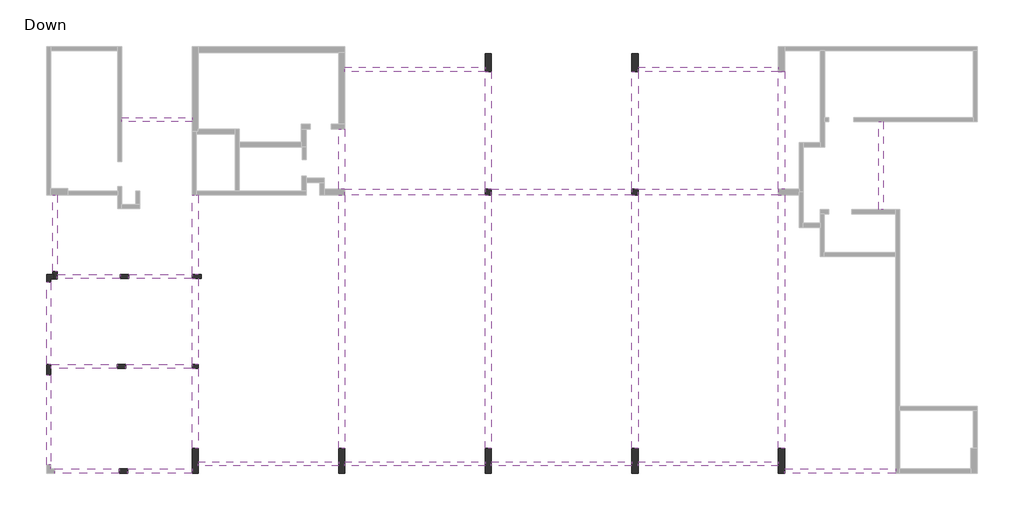
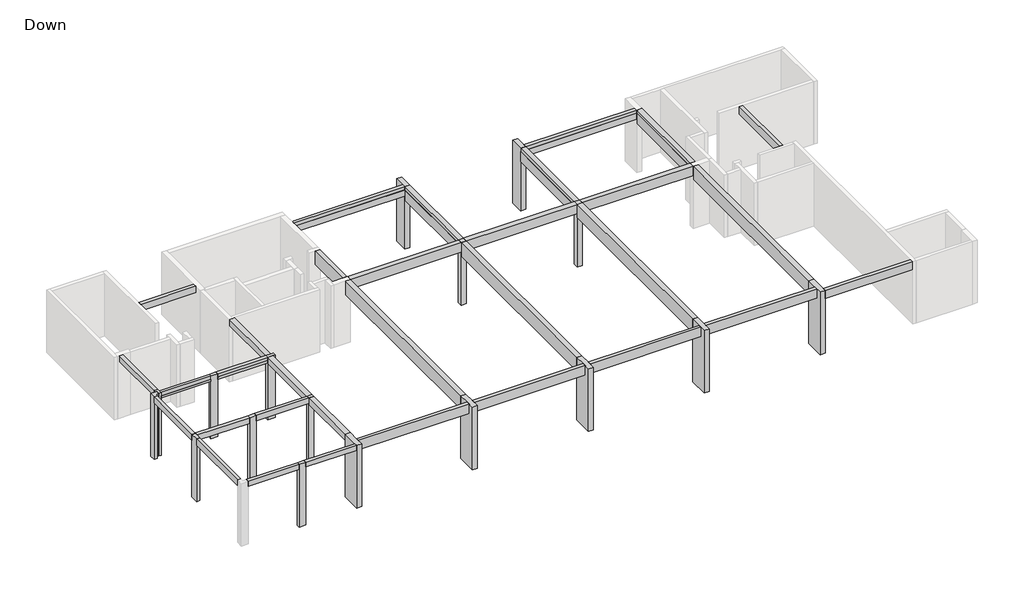
# One storey, part 2 of 2: 32 beams, 17 columns.
"""IFC4 building model written with IfcOpenShell, lengths in millimetres."""

from ifc_helpers import new_model, si_unit, frame, origin, origin_with_axes, place, context, project, spatial, polyline, outline, extrude, faceted_brep, element, save

model = new_model("IFC4")

# Units and contexts
model_context = context("Model", 3, world=origin())
ifc_project = project(units=[si_unit("LENGTHUNIT", "METRE", prefix="MILLI")], contexts=[model_context])

# Site, building, storey
site = spatial("IfcSite", under=ifc_project)
building = spatial("IfcBuilding", under=site)
storey = spatial("IfcBuildingStorey", under=building, Name="Down", Elevation=0.0)

# Beams
placement = place(None, origin())
element("IfcBeam", 1, ObjectType="Concrete Rectengular Beam : 20/30", at=placement, inside=storey, context=model_context, shape_type="Brep", body=[
    faceted_brep([(-13943.2656756, 4006.6682295, 4000.0), (-13943.2656756, 4206.6682295, 4000.0), (-17016.9438365, 4206.6682295, 4000.0), (-17016.9438365, 4006.6682295, 4000.0), (-13943.2656756, 4006.6682295, 3700.0), (-17016.9438365, 4006.6682295, 3700.0), (-13943.2656756, 4206.6682295, 3700.0), (-17016.9438365, 4206.6682295, 3700.0), (-13943.2656756, 4206.6682295, 3790.0)], [[[0, 1, 2, 3]], [[4, 0, 3, 5]], [[6, 4, 5, 7]], [[1, 8, 6, 7, 2]], [[1, 0, 4, 6, 8]], [[3, 2, 7, 5]]]),
])
element("IfcBeam", 2, ObjectType="Concrete Rectengular Beam : 20/30", at=placement, inside=storey, context=model_context, shape_type="SweptSolid", body=[
    extrude(outline(polyline([(-17416.9438365, 4206.6682295), (-17416.9438365, 4006.6682295), (-20492.8250626, 4006.6682295), (-20492.8250626, 4206.6682295), (-17416.9438365, 4206.6682295)])), frame((0.0, 0.0, 3700.0), z_axis=(0.0, 0.0, 1.0), x_axis=(1.0, 0.0, 0.0)), (0.0, 0.0, 1.0), 300.0),
])
element("IfcBeam", 3, ObjectType="Concrete Rectengular Beam : 20/35", at=placement, inside=storey, context=model_context, shape_type="Brep", body=[
    faceted_brep([(-17368.3423039, 13503.9096088, 4000.0), (-20386.1465057, 13503.9096088, 4000.0), (-20386.1465057, 13308.9096088, 4000.0), (-17368.3423039, 13308.9096088, 4000.0), (-20386.1465057, 13303.9096088, 3650.0), (-17368.3423039, 13303.9096088, 3650.0), (-17368.3423039, 13303.9096088, 3790.0), (-20386.1465057, 13303.9096088, 3790.0), (-17368.3423039, 13503.9096088, 3650.0), (-20386.1465057, 13503.9096088, 3650.0), (-20386.1465057, 13503.9096088, 3790.0), (-17368.3423039, 13308.9096088, 3790.0), (-20386.1465057, 13308.9096088, 3790.0)], [[[0, 1, 2, 3]], [[4, 5, 6, 7]], [[8, 5, 4, 9]], [[0, 8, 9, 10, 1]], [[5, 8, 0, 3, 11, 6]], [[9, 4, 7, 12, 2, 1, 10]], [[11, 12, 7, 6]], [[12, 11, 3, 2]]]),
])
element("IfcBeam", 4, ObjectType="Concrete Rectengular Beam : 20/35", at=placement, inside=storey, context=model_context, shape_type="SweptSolid", body=[
    extrude(outline(polyline([(13503.9096088, 3650.0), (13303.9096088, 3650.0), (13303.9096088, 3790.0), (13308.9096088, 3790.0), (13308.9096088, 4000.0), (13503.9096088, 4000.0), (13503.9096088, 3650.0)])), frame((-16968.3423039, 0.0, 0.0), z_axis=(1.0, 0.0, 0.0), x_axis=(0.0, 1.0, 0.0)), (0.0, 0.0, 1.0), 3023.8505747),
])
element("IfcBeam", 5, ObjectType="Concrete Rectengular Beam : 20/35", at=placement, inside=storey, context=model_context, shape_type="Brep", body=[
    faceted_brep([(-20586.1465057, 13648.5145478, 4000.0), (-20386.1465057, 13648.5145478, 4000.0), (-20386.1465057, 17305.3655475, 4000.0), (-20586.1465057, 17305.3655475, 4000.0), (-20386.1465057, 13648.5145478, 3650.0), (-20386.1465057, 17305.3655475, 3650.0), (-20386.1465057, 17305.3655475, 3790.0), (-20586.1465057, 13648.5145478, 3650.0), (-20586.1465057, 17305.3655475, 3650.0)], [[[0, 1, 2, 3]], [[1, 4, 5, 6, 2]], [[4, 7, 8, 5]], [[7, 0, 3, 8]], [[1, 0, 7, 4]], [[3, 2, 6, 5, 8]]]),
])
element("IfcBeam", 6, ObjectType="Concrete Rectengular Beam : 20/35", at=placement, inside=storey, context=model_context, shape_type="SweptSolid", body=[
    extrude(outline(polyline([(-20678.0944112, 9006.6873866), (-20678.0944112, 9206.6873866), (-17516.5223806, 9206.6873866), (-17516.5223806, 9006.6873866), (-20678.0944112, 9006.6873866)])), frame((0.0, 0.0, 3650.0), z_axis=(0.0, 0.0, 1.0), x_axis=(1.0, 0.0, 0.0)), (0.0, 0.0, 1.0), 350.0),
])
element("IfcBeam", 7, ObjectType="Concrete Rectengular Beam : 20/35", at=placement, inside=storey, context=model_context, shape_type="Brep", body=[
    faceted_brep([(-17116.5223806, 9206.6873866, 4000.0), (-17116.5223806, 9006.6873866, 4000.0), (-13943.2656756, 9006.6873866, 4000.0), (-13943.2656756, 9206.6873866, 4000.0), (-17116.5223806, 9006.6873866, 3650.0), (-13943.2656756, 9006.6873866, 3650.0), (-13943.2656756, 9006.6873866, 3790.0), (-17116.5223806, 9206.6873866, 3650.0), (-13943.2656756, 9206.6873866, 3650.0), (-13943.2656756, 9206.6873866, 3790.0)], [[[0, 1, 2, 3]], [[1, 4, 5, 6, 2]], [[4, 7, 8, 5]], [[7, 0, 3, 9, 8]], [[1, 0, 7, 4]], [[2, 6, 5, 8, 9, 3]]]),
])
element("IfcBeam", 8, ObjectType="Concrete Rectengular Beam : 20/40", at=placement, inside=storey, context=model_context, shape_type="Brep", body=[
    faceted_brep([(-20690.7944112, 9206.6873866, 4000.0), (-20890.7944112, 9206.6873866, 4000.0), (-20890.7944112, 9205.6720609, 4000.0), (-20690.7944112, 9205.6720609, 4000.0), (-20690.7944112, 9206.6873866, 3600.0), (-20690.7944112, 9205.6720609, 3600.0), (-20890.7944112, 9206.6873866, 3600.0), (-20890.7944112, 9205.6720609, 3600.0)], [[[0, 1, 2, 3]], [[4, 0, 3, 5]], [[6, 4, 5, 7]], [[1, 6, 7, 2]], [[1, 0, 4, 6]], [[3, 2, 7, 5]]]),
    faceted_brep([(-20890.7944112, 8705.6720609, 4000.0), (-20690.7944112, 8705.6720609, 4000.0), (-20690.7944112, 8705.6720609, 3600.0), (-20890.7944112, 8705.6720609, 3600.0), (-20692.8250626, 4406.6682295, 3600.0), (-20692.8250626, 4406.6682295, 4000.0), (-20890.7944112, 4406.6682295, 4000.0), (-20890.7944112, 4406.6682295, 3600.0), (-20692.8250626, 4206.6682295, 3600.0), (-20692.8250626, 4206.6682295, 4000.0), (-20690.7944112, 4206.6682295, 3600.0), (-20690.7944112, 4206.6682295, 3790.0), (-20690.7944112, 4206.6682295, 4000.0)], [[[0, 1, 2, 3]], [[4, 5, 6, 7]], [[5, 4, 8, 9]], [[9, 8, 10, 11, 12]], [[1, 0, 6, 5, 9, 12]], [[2, 1, 12, 11, 10]], [[3, 2, 10, 8, 4, 7]], [[0, 3, 7, 6]]]),
])
element("IfcBeam", 9, ObjectType="Concrete Rectengular Beam : 20/40", at=placement, inside=storey, context=model_context, shape_type="Brep", body=[
    faceted_brep([(-20890.7944112, 9206.6873866, 4000.0), (-20690.7944112, 9206.6873866, 4000.0), (-20690.7944112, 13148.3800933, 4000.0), (-20890.7944112, 13148.3800933, 4000.0), (-20690.7944112, 9206.6873866, 3790.0), (-20690.7944112, 9206.6873866, 3600.0), (-20690.7944112, 13148.3800933, 3600.0), (-20890.7944112, 9206.6873866, 3600.0), (-20890.7944112, 13148.3800933, 3600.0)], [[[0, 1, 2, 3]], [[1, 4, 5, 6, 2]], [[5, 7, 8, 6]], [[7, 0, 3, 8]], [[3, 2, 6, 8]], [[1, 0, 7, 5, 4]]]),
])
element("IfcBeam", 10, ObjectType="Concrete Rectengular Beam : 20/40", at=placement, inside=storey, context=model_context, shape_type="Brep", body=[
    faceted_brep([(-17292.1354074, 21006.0552027, 4000.0), (-17292.1354074, 20806.0552027, 4000.0), (-13943.2656756, 20806.0552027, 4000.0), (-13943.2656756, 21006.0552027, 4000.0), (-17292.1354074, 20806.0552027, 3790.0), (-17292.1354074, 20806.0552027, 3600.0), (-13943.2656756, 20806.0552027, 3600.0), (-13943.2656756, 20806.0552027, 3790.0), (-17292.1354074, 21006.0552027, 3600.0), (-13943.2656756, 21006.0552027, 3600.0)], [[[0, 1, 2, 3]], [[1, 4, 5, 6, 7, 2]], [[5, 8, 9, 6]], [[8, 0, 3, 9]], [[1, 0, 8, 5, 4]], [[3, 2, 7, 6, 9]]]),
])
element("IfcBeam", 11, ObjectType="Concrete Rectengular Beam : 20/50", at=placement, inside=storey, context=model_context, shape_type="Brep", body=[
    faceted_brep([(14358.5350907, 4204.8099919, 4000.0), (14358.5350907, 4004.8099919, 4000.0), (19658.7266616, 4004.8099919, 4000.0), (19658.7266616, 4204.8099919, 4000.0), (14358.5350907, 4004.8099919, 3500.0), (19658.7266616, 4004.8099919, 3500.0), (14358.5350907, 4204.8099919, 3500.0), (19658.7266616, 4204.8099919, 3500.0), (14358.5350907, 4204.8099919, 3790.0), (19658.7266616, 4204.8099919, 3790.0)], [[[0, 1, 2, 3]], [[1, 4, 5, 2]], [[4, 6, 7, 5]], [[6, 8, 0, 3, 9, 7]], [[1, 0, 8, 6, 4]], [[3, 2, 5, 7, 9]]]),
])
element("IfcBeam", 12, ObjectType="Concrete Rectengular Beam : 20/50", at=placement, inside=storey, context=model_context, shape_type="SweptSolid", body=[
    extrude(outline(polyline([(18864.3013742, 20804.7142065), (19064.3013742, 20804.7142065), (19064.3013742, 16606.2084594), (18864.3013742, 16606.2084594), (18864.3013742, 20804.7142065)])), frame((0.0, 0.0, 3500.0), z_axis=(0.0, 0.0, 1.0), x_axis=(1.0, 0.0, 0.0)), (0.0, 0.0, 1.0), 500.0),
])
element("IfcBeam", 13, ObjectType="Concrete Rectengular Beam : 20/60", at=placement, inside=storey, context=model_context, shape_type="Brep", body=[
    faceted_brep([(58.2285773, 23405.5571184, 4000.0), (-6644.3384725, 23405.5571184, 4000.0), (-6644.3384725, 23225.5571184, 4000.0), (58.2285773, 23225.5571184, 4000.0), (58.2285773, 23405.5571184, 3400.0), (-6644.3384725, 23405.5571184, 3400.0), (58.2285773, 23205.5571184, 3400.0), (-6644.3384725, 23205.5571184, 3400.0), (58.2285773, 23205.5571184, 3790.0), (-6644.3384725, 23205.5571184, 3790.0), (58.2285773, 23225.5571184, 3790.0), (58.2285773, 23206.5724441, 3790.0), (-6644.3384725, 23225.5571184, 3790.0)], [[[0, 1, 2, 3]], [[0, 4, 5, 1]], [[4, 6, 7, 5]], [[7, 6, 8, 9]], [[4, 0, 3, 10, 11, 8, 6]], [[1, 5, 7, 9, 12, 2]], [[10, 12, 9, 8, 11]], [[12, 10, 3, 2]]]),
])
element("IfcBeam", 14, ObjectType="Concrete Rectengular Beam : 20/60", at=placement, inside=storey, context=model_context, shape_type="Brep", body=[
    faceted_brep([(14058.5350907, 23405.5571184, 4000.0), (7356.7343244, 23405.5571184, 4000.0), (7356.7343244, 23210.5571184, 4000.0), (14058.5350907, 23210.5571184, 4000.0), (14358.5350907, 23205.5571184, 3400.0), (14358.5350907, 23205.5571184, 4000.0), (14063.5350907, 23205.5571184, 4000.0), (14063.5350907, 23205.5571184, 3790.0), (14058.5350907, 23205.5571184, 3790.0), (7356.7343244, 23205.5571184, 3790.0), (7356.7343244, 23205.5571184, 3400.0), (14058.5350907, 23205.5571184, 3400.0), (7356.7343244, 23405.5571184, 3400.0), (14058.5350907, 23405.5571184, 3400.0), (14058.5350907, 23206.5724441, 3400.0), (14358.5350907, 23206.5724441, 3400.0), (14358.5350907, 23206.5724441, 4000.0), (7356.7343244, 23206.5724441, 3790.0), (7356.7343244, 23210.5571184, 3790.0), (14058.5350907, 23210.5571184, 3790.0), (14058.5350907, 23206.5724441, 3790.0), (14063.5350907, 23206.5724441, 3790.0), (14063.5350907, 23206.5724441, 4000.0)], [[[0, 1, 2, 3]], [[4, 5, 6, 7, 8, 9, 10, 11]], [[4, 11, 10, 12, 13, 14, 15]], [[12, 1, 0, 13]], [[5, 4, 15, 16]], [[12, 10, 9, 17, 18, 2, 1]], [[14, 13, 0, 3, 19, 20]], [[15, 14, 20, 21, 22, 16]], [[19, 18, 17, 9, 8, 7, 21, 20]], [[21, 7, 6, 22]], [[18, 19, 3, 2]], [[5, 16, 22, 6]]]),
])
element("IfcBeam", 15, ObjectType="Concrete Rectengular Beam : 20/60", at=placement, inside=storey, context=model_context, shape_type="Brep", body=[
    faceted_brep([(7356.7343244, 4552.8176548, 4000.0), (7356.7343244, 4352.8176548, 4000.0), (14058.5350907, 4352.8176548, 4000.0), (14058.5350907, 4552.8176548, 4000.0), (7356.7343244, 4352.8176548, 3400.0), (14058.5350907, 4352.8176548, 3400.0), (7356.7343244, 4552.8176548, 3400.0), (14058.5350907, 4552.8176548, 3400.0), (7356.7343244, 4552.8176548, 3790.0), (14058.5350907, 4552.8176548, 3790.0)], [[[0, 1, 2, 3]], [[1, 4, 5, 2]], [[4, 6, 7, 5]], [[6, 8, 0, 3, 9, 7]], [[1, 0, 8, 6, 4]], [[3, 2, 5, 7, 9]]]),
])
element("IfcBeam", 16, ObjectType="Concrete Rectengular Beam : 20/60", at=placement, inside=storey, context=model_context, shape_type="Brep", body=[
    faceted_brep([(358.2285773, 4552.8176548, 4000.0), (358.2285773, 4352.8176548, 4000.0), (7056.7343244, 4352.8176548, 4000.0), (7056.7343244, 4552.8176548, 4000.0), (358.2285773, 4552.8176548, 3400.0), (358.2285773, 4552.8176548, 3790.0), (7056.7343244, 4552.8176548, 3790.0), (7056.7343244, 4552.8176548, 3400.0), (358.2285773, 4352.8176548, 3400.0), (7056.7343244, 4352.8176548, 3400.0)], [[[0, 1, 2, 3]], [[4, 5, 0, 3, 6, 7]], [[8, 4, 7, 9]], [[1, 8, 9, 2]], [[1, 0, 5, 4, 8]], [[3, 2, 9, 7, 6]]]),
])
element("IfcBeam", 17, ObjectType="Concrete Rectengular Beam : 20/60", at=placement, inside=storey, context=model_context, shape_type="Brep", body=[
    faceted_brep([(-6644.3384725, 4552.8176548, 4000.0), (-6644.3384725, 4352.8176548, 4000.0), (58.2285773, 4352.8176548, 4000.0), (58.2285773, 4552.8176548, 4000.0), (-6644.3384725, 4552.8176548, 3400.0), (-6644.3384725, 4552.8176548, 3790.0), (58.2285773, 4552.8176548, 3790.0), (58.2285773, 4552.8176548, 3400.0), (-6644.3384725, 4352.8176548, 3400.0), (58.2285773, 4352.8176548, 3400.0)], [[[0, 1, 2, 3]], [[4, 5, 0, 3, 6, 7]], [[8, 4, 7, 9]], [[1, 8, 9, 2]], [[1, 0, 5, 4, 8]], [[3, 2, 9, 7, 6]]]),
])
element("IfcBeam", 18, ObjectType="Concrete Rectengular Beam : 20/60", at=placement, inside=storey, context=model_context, shape_type="Brep", body=[
    faceted_brep([(-13643.2656756, 4552.8176548, 4000.0), (-13643.2656756, 4352.8176548, 4000.0), (-6944.3384725, 4352.8176548, 4000.0), (-6944.3384725, 4552.8176548, 4000.0), (-13643.2656756, 4552.8176548, 3400.0), (-13643.2656756, 4552.8176548, 3790.0), (-6944.3384725, 4552.8176548, 3790.0), (-6944.3384725, 4552.8176548, 3400.0), (-13643.2656756, 4352.8176548, 3400.0), (-6944.3384725, 4352.8176548, 3400.0)], [[[0, 1, 2, 3]], [[4, 5, 0, 3, 6, 7]], [[8, 4, 7, 9]], [[1, 8, 9, 2]], [[1, 0, 5, 4, 8]], [[3, 2, 9, 7, 6]]]),
])
element("IfcBeam", 19, ObjectType="Concrete Rectengular Beam : 30/40", at=placement, inside=storey, context=model_context, shape_type="Brep", body=[
    faceted_brep([(-13943.2656756, 13503.9096088, 4000.0), (-13643.2656756, 13503.9096088, 4000.0), (-13643.2656756, 17304.7716778, 4000.0), (-13743.2656756, 17304.7716778, 4000.0), (-13943.2656756, 17304.7716778, 4000.0), (-13643.2656756, 13503.9096088, 3790.0), (-13643.2656756, 13503.9096088, 3600.0), (-13643.2656756, 17304.7716778, 3600.0), (-13643.2656756, 17304.7716778, 3790.0), (-13943.2656756, 13503.9096088, 3600.0), (-13943.2656756, 17304.7716778, 3600.0), (-13943.2656756, 13503.9096088, 3790.0)], [[[0, 1, 2, 3, 4]], [[1, 5, 6, 7, 8, 2]], [[6, 9, 10, 7]], [[9, 11, 0, 4, 10]], [[1, 0, 11, 9, 6, 5]], [[2, 8, 7, 10, 4, 3]]]),
])
element("IfcBeam", 20, ObjectType="Concrete Rectengular Beam : 30/40", at=placement, inside=storey, context=model_context, shape_type="Brep", body=[
    faceted_brep([(-13643.2656756, 13303.9096088, 4000.0), (-13943.2656756, 13303.9096088, 4000.0), (-13943.2656756, 9206.6873866, 4000.0), (-13643.2656756, 9206.6873866, 4000.0), (-13943.2656756, 13303.9096088, 3790.0), (-13943.2656756, 13303.9096088, 3600.0), (-13943.2656756, 9206.6873866, 3600.0), (-13943.2656756, 9206.6873866, 3790.0), (-13643.2656756, 13303.9096088, 3600.0), (-13643.2656756, 9206.6873866, 3600.0), (-13643.2656756, 13303.9096088, 3790.0)], [[[0, 1, 2, 3]], [[1, 4, 5, 6, 7, 2]], [[5, 8, 9, 6]], [[8, 10, 0, 3, 9]], [[8, 5, 4, 1, 0, 10]], [[3, 2, 7, 6, 9]]]),
])
element("IfcBeam", 21, ObjectType="Concrete Rectengular Beam : 30/40", at=placement, inside=storey, context=model_context, shape_type="Brep", body=[
    faceted_brep([(-13943.2656756, 5204.8099919, 4000.0), (-13643.2656756, 5204.8099919, 4000.0), (-13643.2656756, 9006.6873866, 4000.0), (-13943.2656756, 9006.6873866, 4000.0), (-13943.2656756, 5204.8099919, 3600.0), (-13943.2656756, 9006.6873866, 3790.0), (-13943.2656756, 9006.6873866, 3600.0), (-13643.2656756, 5204.8099919, 3600.0), (-13643.2656756, 9006.6873866, 3600.0)], [[[0, 1, 2, 3]], [[4, 0, 3, 5, 6]], [[7, 4, 6, 8]], [[1, 7, 8, 2]], [[1, 0, 4, 7]], [[3, 2, 8, 6, 5]]]),
])
element("IfcBeam", 22, ObjectType="Concrete Rectengular Beam : 30/60", at=placement, inside=storey, context=model_context, shape_type="Brep", body=[
    faceted_brep([(-6644.3384725, 17297.4228975, 4000.0), (58.2285773, 17297.4228975, 4000.0), (58.2285773, 17587.4228975, 4000.0), (-6644.3384725, 17587.4228975, 4000.0), (58.2285773, 17297.4228975, 3400.0), (58.2285773, 17297.4228975, 3790.0), (-6644.3384725, 17297.4228975, 3790.0), (-6644.3384725, 17297.4228975, 3400.0), (58.2285773, 17597.4228975, 3400.0), (-6644.3384725, 17597.4228975, 3400.0), (-6644.3384725, 17597.4228975, 3790.0), (58.2285773, 17597.4228975, 3790.0), (58.2285773, 17587.4228975, 3790.0), (-6644.3384725, 17587.4228975, 3790.0)], [[[0, 1, 2, 3]], [[4, 5, 1, 0, 6, 7]], [[8, 4, 7, 9]], [[8, 9, 10, 11]], [[1, 5, 4, 8, 11, 12, 2]], [[7, 6, 0, 3, 13, 10, 9]], [[13, 12, 11, 10]], [[12, 13, 3, 2]]]),
])
element("IfcBeam", 23, ObjectType="Concrete Rectengular Beam : 30/60", at=placement, inside=storey, context=model_context, shape_type="Brep", body=[
    faceted_brep([(358.2285773, 17597.4228975, 4000.0), (358.2285773, 17297.4228975, 4000.0), (7056.7343244, 17297.4228975, 4000.0), (7056.7343244, 17597.4228975, 4000.0), (358.2285773, 17297.4228975, 3790.0), (358.2285773, 17297.4228975, 3400.0), (7056.7343244, 17297.4228975, 3400.0), (7056.7343244, 17297.4228975, 3790.0), (358.2285773, 17597.4228975, 3400.0), (7056.7343244, 17597.4228975, 3400.0)], [[[0, 1, 2, 3]], [[1, 4, 5, 6, 7, 2]], [[5, 8, 9, 6]], [[8, 0, 3, 9]], [[5, 4, 1, 0, 8]], [[2, 7, 6, 9, 3]]]),
])
element("IfcBeam", 24, ObjectType="Concrete Rectengular Beam : 30/60", at=placement, inside=storey, context=model_context, shape_type="Brep", body=[
    faceted_brep([(7356.7343244, 17297.4228975, 4000.0), (14058.5350907, 17297.4228975, 4000.0), (14058.5350907, 17587.4228975, 4000.0), (7356.7343244, 17587.4228975, 4000.0), (7356.7343244, 17297.4228975, 3790.0), (7356.7343244, 17297.4228975, 3400.0), (14058.5350907, 17297.4228975, 3400.0), (14058.5350907, 17297.4228975, 3790.0), (7356.7343244, 17597.4228975, 3400.0), (14058.5350907, 17597.4228975, 3400.0), (7356.7343244, 17597.4228975, 3790.0), (14058.5350907, 17597.4228975, 3790.0), (7356.7343244, 17587.4228975, 3790.0), (14058.5350907, 17587.4228975, 3790.0)], [[[0, 1, 2, 3]], [[0, 4, 5, 6, 7, 1]], [[5, 8, 9, 6]], [[9, 8, 10, 11]], [[5, 4, 0, 3, 12, 10, 8]], [[6, 9, 11, 13, 2, 1, 7]], [[12, 13, 11, 10]], [[13, 12, 3, 2]]]),
])
element("IfcBeam", 25, ObjectType="Concrete Rectengular Beam : 30/85", at=placement, inside=storey, context=model_context, shape_type="Brep", body=[
    faceted_brep([(-6944.3384725, 20454.6567352, 4000.0), (-6944.3384725, 17597.4228975, 4000.0), (-6674.3384725, 17597.4228975, 4000.0), (-6674.3384725, 20454.6567352, 4000.0), (-6944.3384725, 17597.4228975, 3150.0), (-6944.3384725, 17597.4228975, 3790.0), (-6944.3384725, 20454.6567352, 3790.0), (-6944.3384725, 20454.6567352, 3150.0), (-6644.3384725, 17597.4228975, 3150.0), (-6644.3384725, 20454.6567352, 3150.0), (-6644.3384725, 20454.6567352, 3790.0), (-6644.3384725, 17597.4228975, 3790.0), (-6674.3384725, 17597.4228975, 3790.0), (-6674.3384725, 20454.6567352, 3790.0)], [[[0, 1, 2, 3]], [[4, 5, 1, 0, 6, 7]], [[8, 4, 7, 9]], [[8, 9, 10, 11]], [[1, 5, 4, 8, 11, 12, 2]], [[7, 6, 0, 3, 13, 10, 9]], [[13, 12, 11, 10]], [[12, 13, 3, 2]]]),
])
element("IfcBeam", 26, ObjectType="Concrete Rectengular Beam : 30/85", at=placement, inside=storey, context=model_context, shape_type="Brep", body=[
    faceted_brep([(-6944.3384725, 5204.8099919, 4000.0), (-6644.3384725, 5204.8099919, 4000.0), (-6644.3384725, 17297.4228975, 4000.0), (-6944.3384725, 17297.4228975, 4000.0), (-6944.3384725, 5204.8099919, 3150.0), (-6944.3384725, 17297.4228975, 3790.0), (-6944.3384725, 17297.4228975, 3150.0), (-6644.3384725, 5204.8099919, 3150.0), (-6644.3384725, 17297.4228975, 3150.0), (-6644.3384725, 17297.4228975, 3790.0)], [[[0, 1, 2, 3]], [[4, 0, 3, 5, 6]], [[7, 4, 6, 8]], [[1, 7, 8, 9, 2]], [[1, 0, 4, 7]], [[3, 2, 9, 8, 6, 5]]]),
])
element("IfcBeam", 27, ObjectType="Concrete Rectengular Beam : 30/85", at=placement, inside=storey, context=model_context, shape_type="Brep", body=[
    faceted_brep([(58.2285773, 5204.8099919, 4000.0), (358.2285773, 5204.8099919, 4000.0), (358.2285773, 17297.4228975, 4000.0), (58.2285773, 17297.4228975, 4000.0), (358.2285773, 5204.8099919, 3150.0), (358.2285773, 17297.4228975, 3150.0), (358.2285773, 17297.4228975, 3790.0), (58.2285773, 5204.8099919, 3150.0), (58.2285773, 17297.4228975, 3150.0), (58.2285773, 17297.4228975, 3790.0)], [[[0, 1, 2, 3]], [[1, 4, 5, 6, 2]], [[4, 7, 8, 5]], [[7, 0, 3, 9, 8]], [[1, 0, 7, 4]], [[3, 2, 6, 5, 8, 9]]]),
])
element("IfcBeam", 28, ObjectType="Concrete Rectengular Beam : 30/85", at=placement, inside=storey, context=model_context, shape_type="Brep", body=[
    faceted_brep([(68.2285773, 23206.5724441, 4000.0), (68.2285773, 17597.4228975, 4000.0), (353.2285773, 17597.4228975, 4000.0), (353.2285773, 23206.5724441, 4000.0), (358.2285773, 17597.4228975, 3150.0), (358.2285773, 23206.5724441, 3150.0), (358.2285773, 23206.5724441, 3790.0), (358.2285773, 23205.5571184, 3790.0), (358.2285773, 17597.4228975, 3790.0), (58.2285773, 23206.5724441, 3150.0), (58.2285773, 17597.4228975, 3150.0), (58.2285773, 17597.4228975, 3790.0), (58.2285773, 23205.5571184, 3790.0), (58.2285773, 23206.5724441, 3790.0), (68.2285773, 23206.5724441, 3790.0), (353.2285773, 23206.5724441, 3790.0), (353.2285773, 17597.4228975, 3790.0), (68.2285773, 17597.4228975, 3790.0)], [[[0, 1, 2, 3]], [[4, 5, 6, 7, 8]], [[9, 5, 4, 10]], [[9, 10, 11, 12, 13]], [[5, 9, 13, 14, 0, 3, 15, 6]], [[10, 4, 8, 16, 2, 1, 17, 11]], [[17, 14, 13, 12, 11]], [[14, 17, 1, 0]], [[15, 16, 8, 7, 6]], [[16, 15, 3, 2]]]),
])
element("IfcBeam", 29, ObjectType="Concrete Rectengular Beam : 30/85", at=placement, inside=storey, context=model_context, shape_type="Brep", body=[
    faceted_brep([(7061.7343244, 23206.5724441, 4000.0), (7061.7343244, 17597.4228975, 4000.0), (7351.7343244, 17597.4228975, 4000.0), (7351.7343244, 23206.5724441, 4000.0), (7356.7343244, 17597.4228975, 3150.0), (7356.7343244, 23206.5724441, 3150.0), (7356.7343244, 23206.5724441, 3790.0), (7356.7343244, 23205.5571184, 3790.0), (7356.7343244, 17597.4228975, 3790.0), (7056.7343244, 23206.5724441, 3150.0), (7056.7343244, 17597.4228975, 3150.0), (7056.7343244, 17597.4228975, 3790.0), (7056.7343244, 23205.5571184, 3790.0), (7056.7343244, 23206.5724441, 3790.0), (7061.7343244, 23206.5724441, 3790.0), (7351.7343244, 23206.5724441, 3790.0), (7351.7343244, 17597.4228975, 3790.0), (7061.7343244, 17597.4228975, 3790.0)], [[[0, 1, 2, 3]], [[4, 5, 6, 7, 8]], [[9, 5, 4, 10]], [[9, 10, 11, 12, 13]], [[5, 9, 13, 14, 0, 3, 15, 6]], [[10, 4, 8, 16, 2, 1, 17, 11]], [[17, 14, 13, 12, 11]], [[14, 17, 1, 0]], [[15, 16, 8, 7, 6]], [[16, 15, 3, 2]]]),
])
element("IfcBeam", 30, ObjectType="Concrete Rectengular Beam : 30/85", at=placement, inside=storey, context=model_context, shape_type="Brep", body=[
    faceted_brep([(7056.7343244, 5204.8099919, 4000.0), (7356.7343244, 5204.8099919, 4000.0), (7356.7343244, 17297.4228975, 4000.0), (7056.7343244, 17297.4228975, 4000.0), (7056.7343244, 5204.8099919, 3150.0), (7056.7343244, 17297.4228975, 3790.0), (7056.7343244, 17297.4228975, 3150.0), (7356.7343244, 5204.8099919, 3150.0), (7356.7343244, 17297.4228975, 3150.0), (7356.7343244, 17297.4228975, 3790.0)], [[[0, 1, 2, 3]], [[4, 0, 3, 5, 6]], [[7, 4, 6, 8]], [[1, 7, 8, 9, 2]], [[1, 0, 4, 7]], [[3, 2, 9, 8, 6, 5]]]),
])
element("IfcBeam", 31, ObjectType="Concrete Rectengular Beam : 30/85", at=placement, inside=storey, context=model_context, shape_type="Brep", body=[
    faceted_brep([(14058.5350907, 5204.8099919, 4000.0), (14358.5350907, 5204.8099919, 4000.0), (14358.5350907, 17297.4228975, 4000.0), (14058.5350907, 17297.4228975, 4000.0), (14358.5350907, 5204.8099919, 3150.0), (14358.5350907, 17297.4228975, 3150.0), (14358.5350907, 17297.4228975, 3790.0), (14058.5350907, 5204.8099919, 3150.0), (14058.5350907, 17297.4228975, 3150.0), (14058.5350907, 17297.4228975, 3790.0)], [[[0, 1, 2, 3]], [[1, 4, 5, 6, 2]], [[4, 7, 8, 5]], [[7, 0, 3, 9, 8]], [[1, 0, 7, 4]], [[3, 2, 6, 5, 8, 9]]]),
])
element("IfcBeam", 32, ObjectType="Concrete Rectengular Beam : 30/85", at=placement, inside=storey, context=model_context, shape_type="Brep", body=[
    faceted_brep([(14358.5350907, 17597.4228975, 4000.0), (14358.5350907, 17597.4228975, 3790.0), (14358.5350907, 17597.4228975, 3150.0), (14358.5350907, 23206.5724441, 3150.0), (14358.5350907, 23206.5724441, 3400.0), (14358.5350907, 23205.5571184, 3400.0), (14358.5350907, 23205.5571184, 4000.0), (14058.5350907, 17597.4228975, 3150.0), (14058.5350907, 23206.5724441, 3150.0), (14058.5350907, 17597.4228975, 3790.0), (14058.5350907, 23205.5571184, 3790.0), (14058.5350907, 23205.5571184, 3400.0), (14058.5350907, 23206.5724441, 3400.0), (14063.5350907, 17597.4228975, 4000.0), (14063.5350907, 17597.4228975, 3790.0), (14063.5350907, 23205.5571184, 3790.0), (14063.5350907, 23205.5571184, 4000.0)], [[[0, 1, 2, 3, 4, 5, 6]], [[2, 7, 8, 3]], [[8, 7, 9, 10, 11, 12]], [[2, 1, 0, 13, 14, 9, 7]], [[5, 11, 10, 15, 16, 6]], [[11, 5, 4, 12]], [[0, 6, 16, 13]], [[4, 3, 8, 12]], [[14, 15, 10, 9]], [[15, 14, 13, 16]]]),
])

# Columns
element("IfcColumn", 33, ObjectType="Concrete Rectengular Column : 20/30", at=placement, inside=storey, context=model_context, shape_type="Brep", body=[
    faceted_brep([(-13943.2656756, 9206.6873866, 0.0), (-13643.2656756, 9206.6873866, 0.0), (-13643.2656756, 9006.6873866, 0.0), (-13943.2656756, 9006.6873866, 0.0), (-13943.2656756, 9206.6873866, 4000.0), (-13643.2656756, 9206.6873866, 4000.0), (-13643.2656756, 9206.6873866, 3600.0), (-13943.2656756, 9206.6873866, 3600.0), (-13643.2656756, 9006.6873866, 4000.0), (-13643.2656756, 9006.6873866, 3600.0), (-13943.2656756, 9006.6873866, 4000.0), (-13943.2656756, 9006.6873866, 3600.0)], [[[0, 1, 2, 3]], [[4, 5, 6, 1, 0, 7]], [[5, 8, 9, 2, 1, 6]], [[8, 10, 11, 3, 2, 9]], [[10, 4, 7, 0, 3, 11]], [[4, 10, 8, 5]]]),
])
element("IfcColumn", 34, ObjectType="Concrete Rectengular Column : 20/40", at=placement, inside=storey, context=model_context, shape_type="SweptSolid", body=[
    extrude(outline(polyline([(-17416.9438365, 4206.6682295), (-17016.9438365, 4206.6682295), (-17016.9438365, 4006.6682295), (-17416.9438365, 4006.6682295), (-17416.9438365, 4206.6682295)])), origin_with_axes(), (0.0, 0.0, 1.0), 4000.0),
])
element("IfcColumn", 35, ObjectType="Concrete Rectengular Column : 20/40", at=placement, inside=storey, context=model_context, shape_type="SweptSolid", body=[
    extrude(outline(polyline([(-17516.5223806, 9206.6873866), (-17116.5223806, 9206.6873866), (-17116.5223806, 9006.6873866), (-17516.5223806, 9006.6873866), (-17516.5223806, 9206.6873866)])), origin_with_axes(), (0.0, 0.0, 1.0), 4000.0),
])
element("IfcColumn", 36, ObjectType="Concrete Rectengular Column : 20/40", at=placement, inside=storey, context=model_context, shape_type="Brep", body=[
    faceted_brep([(-17368.3423039, 13503.9096088, 0.0), (-16968.3423039, 13503.9096088, 0.0), (-16968.3423039, 13303.9096088, 0.0), (-17368.3423039, 13303.9096088, 0.0), (-17368.3423039, 13503.9096088, 4000.0), (-16968.3423039, 13503.9096088, 4000.0), (-16968.3423039, 13308.9096088, 4000.0), (-16968.3423039, 13303.9096088, 4000.0), (-16968.3423039, 13303.9096088, 3790.0), (-17368.3423039, 13303.9096088, 4000.0), (-17368.3423039, 13303.9096088, 3790.0), (-17368.3423039, 13308.9096088, 4000.0)], [[[0, 1, 2, 3]], [[4, 5, 1, 0]], [[5, 6, 7, 8, 2, 1]], [[7, 9, 10, 3, 2, 8]], [[9, 11, 4, 0, 3, 10]], [[4, 11, 9, 7, 6, 5]]]),
])
element("IfcColumn", 37, ObjectType="Concrete Rectengular Column : 20/45", at=placement, inside=storey, context=model_context, shape_type="Brep", body=[
    faceted_brep([(-13944.4917292, 13503.9096088, 0.0), (-13494.4917292, 13503.9096088, 0.0), (-13494.4917292, 13303.9096088, 0.0), (-13944.4917292, 13303.9096088, 0.0), (-13944.4917292, 13503.9096088, 4000.0), (-13943.2656756, 13503.9096088, 4000.0), (-13643.2656756, 13503.9096088, 4000.0), (-13494.4917292, 13503.9096088, 4000.0), (-13494.4917292, 13503.9096088, 3790.0), (-13494.4917292, 13303.9096088, 4000.0), (-13494.4917292, 13303.9096088, 3790.0), (-13643.2656756, 13303.9096088, 4000.0), (-13943.2656756, 13303.9096088, 4000.0), (-13944.4917292, 13303.9096088, 4000.0), (-13944.4917292, 13303.9096088, 3790.0), (-13944.4917292, 13308.9096088, 4000.0)], [[[0, 1, 2, 3]], [[4, 5, 6, 7, 8, 1, 0]], [[7, 9, 10, 2, 1, 8]], [[9, 11, 12, 13, 14, 3, 2, 10]], [[13, 15, 4, 0, 3, 14]], [[4, 15, 13, 12, 11, 9, 7, 6, 5]]]),
])
element("IfcColumn", 38, ObjectType="Concrete Rectengular Column : 20/50", at=placement, inside=storey, context=model_context, shape_type="Brep", body=[
    faceted_brep([(-20890.7944112, 8705.6720609, 0.0), (-20890.7944112, 9205.6720609, 0.0), (-20690.7944112, 9205.6720609, 0.0), (-20690.7944112, 8705.6720609, 0.0), (-20890.7944112, 8705.6720609, 4000.0), (-20890.7944112, 9205.6720609, 4000.0), (-20690.7944112, 9205.6720609, 4000.0), (-20690.7944112, 9006.6873866, 4000.0), (-20690.7944112, 8705.6720609, 4000.0)], [[[0, 1, 2, 3]], [[4, 5, 1, 0]], [[5, 6, 2, 1]], [[6, 7, 8, 3, 2]], [[8, 4, 0, 3]], [[4, 8, 7, 6, 5]]]),
])
element("IfcColumn", 39, ObjectType="Concrete Rectengular Column : 30/120", at=placement, inside=storey, context=model_context, shape_type="Brep", body=[
    faceted_brep([(-13643.2656756, 5204.8099919, 0.0), (-13643.2656756, 4004.8099919, 0.0), (-13943.2656756, 4004.8099919, 0.0), (-13943.2656756, 5204.8099919, 0.0), (-13643.2656756, 5204.8099919, 4000.0), (-13643.2656756, 4552.8176548, 4000.0), (-13643.2656756, 4004.8099919, 4000.0), (-13943.2656756, 4004.8099919, 4000.0), (-13943.2656756, 4206.6682295, 4000.0), (-13943.2656756, 5204.8099919, 4000.0)], [[[0, 1, 2, 3]], [[4, 5, 6, 1, 0]], [[6, 7, 2, 1]], [[7, 8, 9, 3, 2]], [[9, 4, 0, 3]], [[4, 9, 8, 7, 6, 5]]]),
])
element("IfcColumn", 40, ObjectType="Concrete Rectengular Column : 30/120", at=placement, inside=storey, context=model_context, shape_type="Brep", body=[
    faceted_brep([(-6644.3384725, 5204.8099919, 0.0), (-6644.3384725, 4004.8099919, 0.0), (-6944.3384725, 4004.8099919, 0.0), (-6944.3384725, 5204.8099919, 0.0), (-6644.3384725, 5204.8099919, 4000.0), (-6644.3384725, 4552.8176548, 4000.0), (-6644.3384725, 4004.8099919, 4000.0), (-6944.3384725, 4004.8099919, 4000.0), (-6944.3384725, 4552.8176548, 4000.0), (-6944.3384725, 5204.8099919, 4000.0)], [[[0, 1, 2, 3]], [[4, 5, 6, 1, 0]], [[6, 7, 2, 1]], [[7, 8, 9, 3, 2]], [[9, 4, 0, 3]], [[4, 9, 8, 7, 6, 5]]]),
])
element("IfcColumn", 41, ObjectType="Concrete Rectengular Column : 30/120", at=placement, inside=storey, context=model_context, shape_type="Brep", body=[
    faceted_brep([(358.2285773, 5204.8099919, 0.0), (358.2285773, 4004.8099919, 0.0), (58.2285773, 4004.8099919, 0.0), (58.2285773, 5204.8099919, 0.0), (358.2285773, 5204.8099919, 4000.0), (358.2285773, 4552.8176548, 4000.0), (358.2285773, 4004.8099919, 4000.0), (58.2285773, 4004.8099919, 4000.0), (58.2285773, 4552.8176548, 4000.0), (58.2285773, 5204.8099919, 4000.0)], [[[0, 1, 2, 3]], [[4, 5, 6, 1, 0]], [[6, 7, 2, 1]], [[7, 8, 9, 3, 2]], [[9, 4, 0, 3]], [[4, 9, 8, 7, 6, 5]]]),
])
element("IfcColumn", 42, ObjectType="Concrete Rectengular Column : 30/120", at=placement, inside=storey, context=model_context, shape_type="Brep", body=[
    faceted_brep([(7356.7343244, 5204.8099919, 0.0), (7356.7343244, 4004.8099919, 0.0), (7056.7343244, 4004.8099919, 0.0), (7056.7343244, 5204.8099919, 0.0), (7356.7343244, 5204.8099919, 4000.0), (7356.7343244, 4552.8176548, 4000.0), (7356.7343244, 4004.8099919, 4000.0), (7056.7343244, 4004.8099919, 4000.0), (7056.7343244, 4552.8176548, 4000.0), (7056.7343244, 5204.8099919, 4000.0)], [[[0, 1, 2, 3]], [[4, 5, 6, 1, 0]], [[6, 7, 2, 1]], [[7, 8, 9, 3, 2]], [[9, 4, 0, 3]], [[4, 9, 8, 7, 6, 5]]]),
])
element("IfcColumn", 43, ObjectType="Concrete Rectengular Column : 30/120", at=placement, inside=storey, context=model_context, shape_type="Brep", body=[
    faceted_brep([(14358.5350907, 5204.8099919, 0.0), (14358.5350907, 4004.8099919, 0.0), (14058.5350907, 4004.8099919, 0.0), (14058.5350907, 5204.8099919, 0.0), (14358.5350907, 5204.8099919, 4000.0), (14358.5350907, 4204.8099919, 4000.0), (14358.5350907, 4004.8099919, 4000.0), (14058.5350907, 4004.8099919, 4000.0), (14058.5350907, 4552.8176548, 4000.0), (14058.5350907, 5204.8099919, 4000.0)], [[[0, 1, 2, 3]], [[4, 5, 6, 1, 0]], [[6, 7, 2, 1]], [[7, 8, 9, 3, 2]], [[9, 4, 0, 3]], [[4, 9, 8, 7, 6, 5]]]),
])
element("IfcColumn", 44, ObjectType="Concrete Rectengular Column : 30/30", at=placement, inside=storey, context=model_context, shape_type="Brep", body=[
    faceted_brep([(358.2285773, 17597.4228975, 0.0), (358.2285773, 17297.4228975, 0.0), (58.2285773, 17297.4228975, 0.0), (58.2285773, 17597.4228975, 0.0), (358.2285773, 17597.4228975, 4000.0), (358.2285773, 17297.4228975, 4000.0), (58.2285773, 17297.4228975, 4000.0), (58.2285773, 17587.4228975, 4000.0), (58.2285773, 17597.4228975, 4000.0), (58.2285773, 17597.4228975, 3790.0), (68.2285773, 17597.4228975, 4000.0), (353.2285773, 17597.4228975, 4000.0)], [[[0, 1, 2, 3]], [[4, 5, 1, 0]], [[5, 6, 2, 1]], [[6, 7, 8, 9, 3, 2]], [[8, 10, 11, 4, 0, 3, 9]], [[4, 11, 10, 8, 7, 6, 5]]]),
])
element("IfcColumn", 45, ObjectType="Concrete Rectengular Column : 30/30", at=placement, inside=storey, context=model_context, shape_type="Brep", body=[
    faceted_brep([(7356.7343244, 17597.4228975, 0.0), (7356.7343244, 17297.4228975, 0.0), (7056.7343244, 17297.4228975, 0.0), (7056.7343244, 17597.4228975, 0.0), (7356.7343244, 17597.4228975, 4000.0), (7356.7343244, 17587.4228975, 4000.0), (7356.7343244, 17297.4228975, 4000.0), (7356.7343244, 17597.4228975, 3790.0), (7056.7343244, 17297.4228975, 4000.0), (7056.7343244, 17597.4228975, 4000.0), (7061.7343244, 17597.4228975, 4000.0), (7351.7343244, 17597.4228975, 4000.0)], [[[0, 1, 2, 3]], [[4, 5, 6, 1, 0, 7]], [[6, 8, 2, 1]], [[8, 9, 3, 2]], [[9, 10, 11, 4, 7, 0, 3]], [[4, 11, 10, 9, 8, 6, 5]]]),
])
element("IfcColumn", 46, ObjectType="Concrete Rectengular Column : 30/85", at=placement, inside=storey, context=model_context, shape_type="Brep", body=[
    faceted_brep([(358.2285773, 24056.5724441, 0.0), (358.2285773, 23206.5724441, 0.0), (58.2285773, 23206.5724441, 0.0), (58.2285773, 24056.5724441, 0.0), (358.2285773, 24056.5724441, 4000.0), (358.2285773, 23405.5571184, 4000.0), (358.2285773, 23210.5571184, 4000.0), (358.2285773, 23206.5724441, 4000.0), (358.2285773, 23206.5724441, 3790.0), (353.2285773, 23206.5724441, 4000.0), (68.2285773, 23206.5724441, 4000.0), (58.2285773, 23206.5724441, 4000.0), (58.2285773, 23206.5724441, 3790.0), (58.2285773, 23225.5571184, 4000.0), (58.2285773, 24056.5724441, 4000.0)], [[[0, 1, 2, 3]], [[4, 5, 6, 7, 8, 1, 0]], [[7, 9, 10, 11, 12, 2, 1, 8]], [[11, 13, 14, 3, 2, 12]], [[14, 4, 0, 3]], [[4, 14, 13, 11, 10, 9, 7, 6, 5]]]),
])
element("IfcColumn", 47, ObjectType="Concrete Rectengular Column : 30/85", at=placement, inside=storey, context=model_context, shape_type="Brep", body=[
    faceted_brep([(7356.7343244, 24056.5724441, 0.0), (7356.7343244, 23206.5724441, 0.0), (7056.7343244, 23206.5724441, 0.0), (7056.7343244, 24056.5724441, 0.0), (7356.7343244, 24056.5724441, 4000.0), (7356.7343244, 23210.5571184, 4000.0), (7356.7343244, 23206.5724441, 4000.0), (7356.7343244, 23206.5724441, 3790.0), (7351.7343244, 23206.5724441, 4000.0), (7061.7343244, 23206.5724441, 4000.0), (7056.7343244, 23206.5724441, 4000.0), (7056.7343244, 23206.5724441, 3790.0), (7056.7343244, 23210.5571184, 4000.0), (7056.7343244, 24056.5724441, 4000.0)], [[[0, 1, 2, 3]], [[4, 5, 6, 7, 1, 0]], [[6, 8, 9, 10, 11, 2, 1, 7]], [[10, 12, 13, 3, 2, 11]], [[13, 4, 0, 3]], [[4, 13, 12, 10, 9, 8, 6, 5]]]),
])
element("IfcColumn", 48, ObjectType="L Column : 35/35/20/20", at=placement, inside=storey, context=model_context, shape_type="Brep", body=[
    faceted_brep([(-20890.7944112, 13498.3800933, 0.0), (-20586.1465057, 13498.3800933, 0.0), (-20540.7944112, 13498.3800933, 0.0), (-20540.7944112, 13298.3800933, 0.0), (-20690.7944112, 13298.3800933, 0.0), (-20690.7944112, 13148.3800933, 0.0), (-20890.7944112, 13148.3800933, 0.0), (-20890.7944112, 13498.3800933, 4000.0), (-20586.1465057, 13498.3800933, 4000.0), (-20540.7944112, 13498.3800933, 4000.0), (-20540.7944112, 13298.3800933, 4000.0), (-20690.7944112, 13298.3800933, 4000.0), (-20690.7944112, 13298.3800933, 3790.0), (-20690.7944112, 13148.3800933, 4000.0), (-20890.7944112, 13148.3800933, 4000.0)], [[[0, 1, 2, 3, 4, 5, 6]], [[7, 8, 9, 2, 1, 0]], [[9, 10, 3, 2]], [[10, 11, 12, 4, 3]], [[11, 13, 5, 4, 12]], [[13, 14, 6, 5]], [[14, 7, 0, 6]], [[7, 14, 13, 11, 10, 9, 8]]]),
])
element("IfcColumn", 49, ObjectType="L Column : 35/35/20/20", at=placement, inside=storey, context=model_context, shape_type="Brep", body=[
    faceted_brep([(-20586.1465057, 13498.5145478, 0.0), (-20586.1465057, 13648.5145478, 0.0), (-20386.1465057, 13648.5145478, 0.0), (-20386.1465057, 13298.5145478, 0.0), (-20540.7944112, 13298.5145478, 0.0), (-20540.7944112, 13498.3800933, 0.0), (-20386.1465057, 13298.5145478, 3790.0), (-20386.1465057, 13298.5145478, 4000.0), (-20540.7944112, 13298.5145478, 4000.0), (-20586.1465057, 13498.3800933, 4000.0), (-20586.1465057, 13648.5145478, 4000.0), (-20386.1465057, 13648.5145478, 4000.0), (-20386.1465057, 13503.9096088, 4000.0), (-20386.1465057, 13308.9096088, 4000.0), (-20540.7944112, 13498.3800933, 4000.0)], [[[0, 1, 2, 3, 4, 5]], [[3, 6, 7, 8, 4]], [[1, 0, 9, 10]], [[2, 1, 10, 11]], [[3, 2, 11, 12, 13, 7, 6]], [[10, 9, 14, 8, 7, 13, 12, 11]], [[5, 14, 9, 0]], [[14, 5, 4, 8]]]),
])

save(model, "model.ifc")

# Revit data of these elements
# Type "Concrete Rectengular Beam : 20/30"
#   Length [instance default] = 152.4 cm
#   b = 20 cm
#   h = 30 cm
#   Structural Material [instance default] = Concrete
#   Assembly Code = ""
# Type "Concrete Rectengular Beam : 20/35"
#   Length [instance default] = 152.4 cm
#   b = 20 cm
#   h = 35 cm
#   Structural Material [instance default] = Concrete
#   Assembly Code = ""
# Type "Concrete Rectengular Beam : 20/40"
#   Keynote = "09000"
#   Length [instance default] = 152.4 cm
#   b = 20 cm
#   h = 40 cm
#   Structural Material [instance default] = Concrete
#   Assembly Code = ""
# Type "Concrete Rectengular Beam : 20/50"
#   Length [instance default] = 152.4 cm
#   b = 20 cm
#   h = 50 cm
#   Structural Material [instance default] = Concrete
#   Assembly Code = ""
# Type "Concrete Rectengular Beam : 20/60"
#   Length [instance default] = 152.4 cm
#   b = 20 cm
#   h = 60 cm
#   Structural Material [instance default] = Concrete
#   Assembly Code = ""
# Type "Concrete Rectengular Beam : 30/40"
#   Length [instance default] = 152.4 cm
#   b = 30 cm
#   h = 40 cm
#   Structural Material [instance default] = Concrete
#   Assembly Code = ""
# Type "Concrete Rectengular Beam : 30/60"
#   Length [instance default] = 152.4 cm
#   b = 30 cm
#   h = 60 cm
#   Structural Material [instance default] = Concrete
#   Assembly Code = ""
# Type "Concrete Rectengular Beam : 30/85"
#   Length [instance default] = 152.4 cm
#   b = 30 cm
#   h = 85 cm
#   Structural Material [instance default] = Concrete
#   Assembly Code = ""
# Type "Concrete Rectengular Column : 20/30"
#   b = 20 cm
#   h = 30 cm
#   Structural Material [instance default] = Concrete
# Type "Concrete Rectengular Column : 20/40"
#   b = 20 cm
#   h = 40 cm
#   Structural Material [instance default] = Concrete
# Type "Concrete Rectengular Column : 20/45"
#   b = 20 cm
#   h = 45 cm
#   Structural Material [instance default] = Concrete
# Type "Concrete Rectengular Column : 20/50"
#   b = 20 cm
#   h = 50 cm
#   Structural Material [instance default] = Concrete
# Type "Concrete Rectengular Column : 30/120"
#   b = 30 cm
#   h = 120 cm
#   Structural Material [instance default] = Concrete
# Type "Concrete Rectengular Column : 30/30"
#   b = 30 cm
#   h = 30 cm
#   Structural Material [instance default] = Concrete
# Type "Concrete Rectengular Column : 30/85"
#   b = 30 cm
#   h = 85 cm
#   Structural Material [instance default] = Concrete
# Type "L Column : 35/35/20/20"
#   Small Length = 20 cm
#   Small Depth = 20 cm
#   Depth = 35 cm
#   Length = 35 cm
#   Centroid Y = 70 cm
#   Centroid X = 10 cm
#   Structural Material [instance default] = Concrete, Cast-in-Place gray
# Element 1 (IfcBeam, "Concrete Rectengular Beam : 20/30")
#   Comments = ""
#   Mark = "B1"
#   SOFiSTiK_AMG_Comments = ""
#   SOFiSTiK_AMG_Scheduled = yes
#   SOFiSTiK_AMG_Adjusted = yes
#   Structural Material = Concrete
#   Phase Created = New Construction
#   Materials on its faces: "Concrete"
# Element 2 (IfcBeam, "Concrete Rectengular Beam : 20/30")
#   Comments = ""
#   Mark = "B2"
#   SOFiSTiK_AMG_Comments = ""
#   SOFiSTiK_AMG_Scheduled = yes
#   SOFiSTiK_AMG_Adjusted = yes
#   Structural Material = Concrete
#   Phase Created = New Construction
#   Materials on its faces: "Concrete"
# Element 3 (IfcBeam, "Concrete Rectengular Beam : 20/35")
#   Comments = ""
#   Mark = "B3"
#   SOFiSTiK_AMG_Comments = ""
#   SOFiSTiK_AMG_Scheduled = yes
#   SOFiSTiK_AMG_Adjusted = yes
#   Structural Material = Concrete
#   Phase Created = New Construction
#   Materials on its faces: "Concrete"
# Element 4 (IfcBeam, "Concrete Rectengular Beam : 20/35")
#   Comments = ""
#   Mark = "B4"
#   SOFiSTiK_AMG_Comments = ""
#   SOFiSTiK_AMG_Scheduled = yes
#   SOFiSTiK_AMG_Adjusted = yes
#   Structural Material = Concrete
#   Phase Created = New Construction
#   Materials on its faces: "Concrete"
# Element 5 (IfcBeam, "Concrete Rectengular Beam : 20/35")
#   Comments = ""
#   Mark = "B5"
#   SOFiSTiK_AMG_Comments = ""
#   SOFiSTiK_AMG_Scheduled = yes
#   SOFiSTiK_AMG_Adjusted = yes
#   Structural Material = Concrete
#   Phase Created = New Construction
#   Materials on its faces: "Concrete"
# Element 6 (IfcBeam, "Concrete Rectengular Beam : 20/35")
#   Comments = ""
#   Mark = "B6"
#   SOFiSTiK_AMG_Comments = ""
#   SOFiSTiK_AMG_Scheduled = yes
#   SOFiSTiK_AMG_Adjusted = yes
#   Structural Material = Concrete
#   Phase Created = New Construction
#   Materials on its faces: "Concrete"
# Element 7 (IfcBeam, "Concrete Rectengular Beam : 20/35")
#   Comments = ""
#   Mark = "B7"
#   SOFiSTiK_AMG_Comments = ""
#   SOFiSTiK_AMG_Scheduled = yes
#   SOFiSTiK_AMG_Adjusted = yes
#   Structural Material = Concrete
#   Phase Created = New Construction
#   Materials on its faces: "Concrete"
# Element 8 (IfcBeam, "Concrete Rectengular Beam : 20/40")
#   Comments = ""
#   Mark = "B8"
#   SOFiSTiK_AMG_Comments = ""
#   SOFiSTiK_AMG_Scheduled = yes
#   SOFiSTiK_AMG_Adjusted = yes
#   Structural Material = Concrete
#   Phase Created = New Construction
#   Materials on its faces: "Concrete"
# Element 9 (IfcBeam, "Concrete Rectengular Beam : 20/40")
#   Comments = ""
#   Mark = "B9"
#   SOFiSTiK_AMG_Comments = ""
#   SOFiSTiK_AMG_Scheduled = yes
#   SOFiSTiK_AMG_Adjusted = yes
#   Structural Material = Concrete
#   Phase Created = New Construction
#   Materials on its faces: "Concrete"
# Element 10 (IfcBeam, "Concrete Rectengular Beam : 20/40")
#   Comments = ""
#   Mark = "B10"
#   SOFiSTiK_AMG_Comments = ""
#   SOFiSTiK_AMG_Scheduled = yes
#   SOFiSTiK_AMG_Adjusted = yes
#   Structural Material = Concrete
#   Phase Created = New Construction
#   Materials on its faces: "Concrete"
# Element 11 (IfcBeam, "Concrete Rectengular Beam : 20/50")
#   Comments = ""
#   Mark = "B11"
#   SOFiSTiK_AMG_Comments = ""
#   SOFiSTiK_AMG_Scheduled = yes
#   SOFiSTiK_AMG_Adjusted = yes
#   Structural Material = Concrete
#   Phase Created = New Construction
#   Materials on its faces: "Concrete"
# Element 12 (IfcBeam, "Concrete Rectengular Beam : 20/50")
#   Comments = ""
#   Mark = "B12"
#   SOFiSTiK_AMG_Comments = ""
#   SOFiSTiK_AMG_Scheduled = yes
#   SOFiSTiK_AMG_Adjusted = yes
#   Structural Material = Concrete
#   Phase Created = New Construction
#   Materials on its faces: "Concrete"
# Element 13 (IfcBeam, "Concrete Rectengular Beam : 20/60")
#   Comments = ""
#   Mark = "B13"
#   SOFiSTiK_AMG_Comments = ""
#   SOFiSTiK_AMG_Scheduled = yes
#   SOFiSTiK_AMG_Adjusted = yes
#   Structural Material = Concrete
#   Phase Created = New Construction
#   Materials on its faces: "Concrete"
# Element 14 (IfcBeam, "Concrete Rectengular Beam : 20/60")
#   Comments = ""
#   Mark = "B15"
#   SOFiSTiK_AMG_Comments = ""
#   SOFiSTiK_AMG_Scheduled = yes
#   SOFiSTiK_AMG_Adjusted = yes
#   Structural Material = Concrete
#   Phase Created = New Construction
#   Materials on its faces: "Concrete"
# Element 15 (IfcBeam, "Concrete Rectengular Beam : 20/60")
#   Comments = ""
#   Mark = "B16"
#   SOFiSTiK_AMG_Comments = ""
#   SOFiSTiK_AMG_Scheduled = yes
#   SOFiSTiK_AMG_Adjusted = yes
#   Structural Material = Concrete
#   Phase Created = New Construction
#   Materials on its faces: "Concrete"
# Element 16 (IfcBeam, "Concrete Rectengular Beam : 20/60")
#   Comments = ""
#   Mark = "B17"
#   SOFiSTiK_AMG_Comments = ""
#   SOFiSTiK_AMG_Scheduled = yes
#   SOFiSTiK_AMG_Adjusted = yes
#   Structural Material = Concrete
#   Phase Created = New Construction
#   Materials on its faces: "Concrete"
# Element 17 (IfcBeam, "Concrete Rectengular Beam : 20/60")
#   Comments = ""
#   Mark = "B18"
#   SOFiSTiK_AMG_Comments = ""
#   SOFiSTiK_AMG_Scheduled = yes
#   SOFiSTiK_AMG_Adjusted = yes
#   Structural Material = Concrete
#   Phase Created = New Construction
#   Materials on its faces: "Concrete"
# Element 18 (IfcBeam, "Concrete Rectengular Beam : 20/60")
#   Comments = ""
#   Mark = "B19"
#   SOFiSTiK_AMG_Comments = ""
#   SOFiSTiK_AMG_Scheduled = yes
#   SOFiSTiK_AMG_Adjusted = yes
#   Structural Material = Concrete
#   Phase Created = New Construction
#   Materials on its faces: "Concrete"
# Element 19 (IfcBeam, "Concrete Rectengular Beam : 30/40")
#   Comments = ""
#   Mark = "B20"
#   SOFiSTiK_AMG_Comments = ""
#   SOFiSTiK_AMG_Scheduled = yes
#   SOFiSTiK_AMG_Adjusted = yes
#   Structural Material = Concrete
#   Phase Created = New Construction
#   Materials on its faces: "Concrete"
# Element 20 (IfcBeam, "Concrete Rectengular Beam : 30/40")
#   Comments = ""
#   Mark = "B21"
#   SOFiSTiK_AMG_Comments = ""
#   SOFiSTiK_AMG_Scheduled = yes
#   SOFiSTiK_AMG_Adjusted = yes
#   Structural Material = Concrete
#   Phase Created = New Construction
#   Materials on its faces: "Concrete"
# Element 21 (IfcBeam, "Concrete Rectengular Beam : 30/40")
#   Comments = ""
#   Mark = "B22"
#   SOFiSTiK_AMG_Comments = ""
#   SOFiSTiK_AMG_Scheduled = yes
#   SOFiSTiK_AMG_Adjusted = yes
#   Structural Material = Concrete
#   Phase Created = New Construction
#   Materials on its faces: "Concrete"
# Element 22 (IfcBeam, "Concrete Rectengular Beam : 30/60")
#   Comments = ""
#   Mark = "B23"
#   SOFiSTiK_AMG_Comments = ""
#   SOFiSTiK_AMG_Scheduled = yes
#   SOFiSTiK_AMG_Adjusted = yes
#   Structural Material = Concrete
#   Phase Created = New Construction
#   Materials on its faces: "Concrete"
# Element 23 (IfcBeam, "Concrete Rectengular Beam : 30/60")
#   Comments = ""
#   Mark = "B24"
#   SOFiSTiK_AMG_Comments = ""
#   SOFiSTiK_AMG_Scheduled = yes
#   SOFiSTiK_AMG_Adjusted = yes
#   Structural Material = Concrete
#   Phase Created = New Construction
#   Materials on its faces: "Concrete"
# Element 24 (IfcBeam, "Concrete Rectengular Beam : 30/60")
#   Comments = ""
#   Mark = "B25"
#   SOFiSTiK_AMG_Comments = ""
#   SOFiSTiK_AMG_Scheduled = yes
#   SOFiSTiK_AMG_Adjusted = yes
#   Structural Material = Concrete
#   Phase Created = New Construction
#   Materials on its faces: "Concrete"
# Element 25 (IfcBeam, "Concrete Rectengular Beam : 30/85")
#   Comments = ""
#   Mark = "B26"
#   SOFiSTiK_AMG_Comments = ""
#   SOFiSTiK_AMG_Scheduled = yes
#   SOFiSTiK_AMG_Adjusted = yes
#   Structural Material = Concrete
#   Phase Created = New Construction
#   Materials on its faces: "Concrete"
# Element 26 (IfcBeam, "Concrete Rectengular Beam : 30/85")
#   Comments = ""
#   Mark = "B27"
#   SOFiSTiK_AMG_Comments = ""
#   SOFiSTiK_AMG_Scheduled = yes
#   SOFiSTiK_AMG_Adjusted = yes
#   Structural Material = Concrete
#   Phase Created = New Construction
#   Materials on its faces: "Concrete"
# Element 27 (IfcBeam, "Concrete Rectengular Beam : 30/85")
#   Comments = ""
#   Mark = "B28"
#   SOFiSTiK_AMG_Comments = ""
#   SOFiSTiK_AMG_Scheduled = yes
#   SOFiSTiK_AMG_Adjusted = yes
#   Structural Material = Concrete
#   Phase Created = New Construction
#   Materials on its faces: "Concrete"
# Element 28 (IfcBeam, "Concrete Rectengular Beam : 30/85")
#   Comments = ""
#   Mark = "B29"
#   SOFiSTiK_AMG_Comments = ""
#   SOFiSTiK_AMG_Scheduled = yes
#   SOFiSTiK_AMG_Adjusted = yes
#   Structural Material = Concrete
#   Phase Created = New Construction
#   Materials on its faces: "Concrete"
# Element 29 (IfcBeam, "Concrete Rectengular Beam : 30/85")
#   Comments = ""
#   Mark = "B30"
#   SOFiSTiK_AMG_Comments = ""
#   SOFiSTiK_AMG_Scheduled = yes
#   SOFiSTiK_AMG_Adjusted = yes
#   Structural Material = Concrete
#   Phase Created = New Construction
#   Materials on its faces: "Concrete"
# Element 30 (IfcBeam, "Concrete Rectengular Beam : 30/85")
#   Comments = ""
#   Mark = "B31"
#   SOFiSTiK_AMG_Comments = ""
#   SOFiSTiK_AMG_Scheduled = yes
#   SOFiSTiK_AMG_Adjusted = yes
#   Structural Material = Concrete
#   Phase Created = New Construction
#   Materials on its faces: "Concrete"
# Element 31 (IfcBeam, "Concrete Rectengular Beam : 30/85")
#   Comments = ""
#   Mark = "B32"
#   SOFiSTiK_AMG_Comments = ""
#   SOFiSTiK_AMG_Scheduled = yes
#   SOFiSTiK_AMG_Adjusted = yes
#   Structural Material = Concrete
#   Phase Created = New Construction
#   Materials on its faces: "Concrete"
# Element 32 (IfcBeam, "Concrete Rectengular Beam : 30/85")
#   Comments = ""
#   Mark = "B33"
#   SOFiSTiK_AMG_Comments = ""
#   SOFiSTiK_AMG_Scheduled = yes
#   SOFiSTiK_AMG_Adjusted = yes
#   Structural Material = Concrete
#   Phase Created = New Construction
#   Materials on its faces: "Concrete"
# Element 33 (IfcColumn, "Concrete Rectengular Column : 20/30")
#   Comments = ""
#   Mark = "C1"
#   SOFiSTiK_AMG_Comments = ""
#   SOFiSTiK_AMG_Scheduled = yes
#   SOFiSTiK_AMG_Adjusted = yes
#   Structural Material = Concrete
#   Phase Created = New Construction
#   Materials on its faces: "Concrete"
# Element 34 (IfcColumn, "Concrete Rectengular Column : 20/40")
#   Comments = ""
#   Mark = "C2"
#   SOFiSTiK_AMG_Comments = ""
#   SOFiSTiK_AMG_Scheduled = yes
#   SOFiSTiK_AMG_Adjusted = yes
#   Structural Material = Concrete
#   Phase Created = New Construction
#   Materials on its faces: "Concrete"
# Element 35 (IfcColumn, "Concrete Rectengular Column : 20/40")
#   Comments = ""
#   Mark = "C3"
#   SOFiSTiK_AMG_Comments = ""
#   SOFiSTiK_AMG_Scheduled = yes
#   SOFiSTiK_AMG_Adjusted = yes
#   Structural Material = Concrete
#   Phase Created = New Construction
#   Materials on its faces: "Concrete"
# Element 36 (IfcColumn, "Concrete Rectengular Column : 20/40")
#   Comments = ""
#   Mark = "C4"
#   SOFiSTiK_AMG_Comments = ""
#   SOFiSTiK_AMG_Scheduled = yes
#   SOFiSTiK_AMG_Adjusted = yes
#   Structural Material = Concrete
#   Phase Created = New Construction
#   Materials on its faces: "Concrete"
# Element 37 (IfcColumn, "Concrete Rectengular Column : 20/45")
#   Comments = ""
#   Mark = "C5"
#   SOFiSTiK_AMG_Comments = ""
#   SOFiSTiK_AMG_Scheduled = yes
#   SOFiSTiK_AMG_Adjusted = yes
#   Structural Material = Concrete
#   Phase Created = New Construction
#   Materials on its faces: "Concrete"
# Element 38 (IfcColumn, "Concrete Rectengular Column : 20/50")
#   Comments = ""
#   Mark = "C6"
#   SOFiSTiK_AMG_Comments = ""
#   SOFiSTiK_AMG_Scheduled = yes
#   SOFiSTiK_AMG_Adjusted = yes
#   Structural Material = Concrete
#   Phase Created = New Construction
#   Materials on its faces: "Concrete"
# Element 39 (IfcColumn, "Concrete Rectengular Column : 30/120")
#   Comments = ""
#   Mark = "C7"
#   SOFiSTiK_AMG_Comments = ""
#   SOFiSTiK_AMG_Scheduled = yes
#   SOFiSTiK_AMG_Adjusted = yes
#   Structural Material = Concrete
#   Phase Created = New Construction
#   Materials on its faces: "Concrete"
# Element 40 (IfcColumn, "Concrete Rectengular Column : 30/120")
#   Comments = ""
#   Mark = "C8"
#   SOFiSTiK_AMG_Comments = ""
#   SOFiSTiK_AMG_Scheduled = yes
#   SOFiSTiK_AMG_Adjusted = yes
#   Structural Material = Concrete
#   Phase Created = New Construction
#   Materials on its faces: "Concrete"
# Element 41 (IfcColumn, "Concrete Rectengular Column : 30/120")
#   Comments = ""
#   Mark = "C9"
#   SOFiSTiK_AMG_Comments = ""
#   SOFiSTiK_AMG_Scheduled = yes
#   SOFiSTiK_AMG_Adjusted = yes
#   Structural Material = Concrete
#   Phase Created = New Construction
